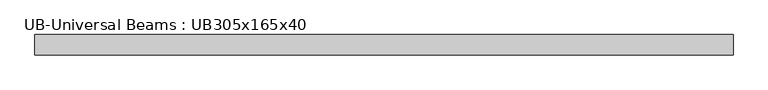
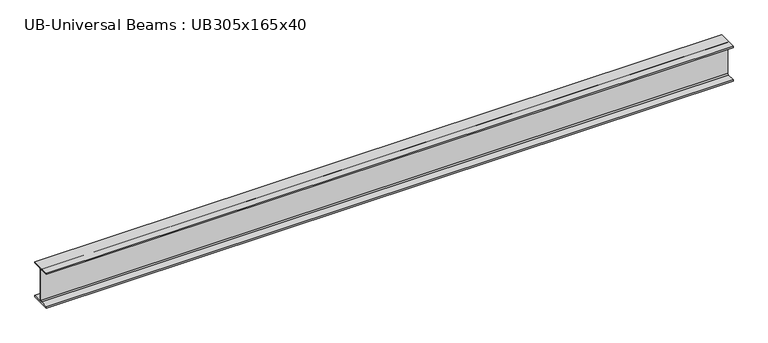
"""IFC4 building model written with IfcOpenShell, lengths in millimetres: beam geometry, UB-Universal Beams : UB305x165x40."""

from ifc_helpers import new_model, si_unit, point, frame, frame_2d, origin, place, context, project, spatial, polyline, circle_curve, trimmed, segment, composite_curve, outline, extrude, source, transform, mapped, element, save


def ub_universal_beams_ub305x165x40_7f5f946b(model_context):
    return source(origin(), model_context, "Body", "SweptSolid", [
        extrude(outline(composite_curve([segment(polyline([(82.5, -141.5), (82.5, -151.7), (-82.5, -151.7), (-82.5, -141.5), (-11.9, -141.5)]), True, "CONTINUOUS"), segment(trimmed(circle_curve(frame_2d((-11.9, -132.6)), 8.9), [point((-11.9, -141.5))], [point((-3.0, -132.6))], True, "CARTESIAN"), True, "CONTINUOUS"), segment(polyline([(-3.0, -132.6), (-3.0, 132.6)]), True, "CONTINUOUS"), segment(trimmed(circle_curve(frame_2d((-11.9, 132.6)), 8.9), [point((-3.0, 132.6))], [point((-11.9, 141.5))], True, "CARTESIAN"), True, "CONTINUOUS"), segment(polyline([(-11.9, 141.5), (-82.5, 141.5), (-82.5, 151.7), (82.5, 151.7), (82.5, 141.5), (11.9, 141.5)]), True, "CONTINUOUS"), segment(trimmed(circle_curve(frame_2d((11.9, 132.6)), 8.9), [point((11.9, 141.5))], [point((3.0, 132.6))], True, "CARTESIAN"), True, "CONTINUOUS"), segment(polyline([(3.0, 132.6), (3.0, -132.6)]), True, "CONTINUOUS"), segment(trimmed(circle_curve(frame_2d((11.9, -132.6)), 8.9), [point((3.0, -132.6))], [point((11.9, -141.5))], True, "CARTESIAN"), True, "CONTINUOUS"), segment(polyline([(11.9, -141.5), (82.5, -141.5)]), True, "CONTINUOUS")], self_intersect=False)), frame((-2833.3, 0.0, 0.0), z_axis=(1.0, 0.0, 0.0), x_axis=(0.0, 1.0, 0.0)), (0.0, 0.0, 1.0), 5666.6),
    ])


if __name__ == "__main__":
    model = new_model("IFC4")
    model_context = context("Model", 3, world=origin())
    ifc_project = project(units=[si_unit("LENGTHUNIT", "METRE", prefix="MILLI")], contexts=[model_context])
    site = spatial("IfcSite", under=ifc_project)
    building = spatial("IfcBuilding", under=site)
    placement = place(None, origin())
    ub_universal_beams_ub305x165x40_shape = ub_universal_beams_ub305x165x40_7f5f946b(model_context)
    element("IfcBeam", 1, ObjectType="UB-Universal Beams : UB305x165x40", at=placement, inside=building, context=model_context, shape_type="MappedRepresentation", body=[
        mapped(ub_universal_beams_ub305x165x40_shape, transform((0.0, 0.0, 0.0), x_axis=(1.0, 0.0, 0.0), y_axis=(0.0, 1.0, 0.0), z_axis=(0.0, 0.0, 1.0))),
    ])
    save(model, "model.ifc")

# Revit data of these elements
# Type "UB-Universal Beams : UB305x165x40"
#   Section Name Key = "UB305X165X40"
#   Width = 16.5 cm
#   Web Thickness = 0.6 cm
#   Web Fillet = 0.89 cm
#   Warping Constant = 164000.0 cm⁶
#   Torsional Moment of Inertia = 14.70 cm⁴
#   Section Area = 51.3 cm²
#   Plastic Modulus weak axis = 142.0 cm³
#   Plastic Modulus strong axis = 623.0 cm³
#   Nominal Weight = 40.2999 kgf/m
#   Moment of Inertia weak axis = 764.00 cm⁴
#   Moment of Inertia strong axis = 8503.00 cm⁴
#   Height = 30.34 cm
#   Flange Thickness = 1.02 cm
#   Elastic Modulus weak axis = 92.6 cm³
#   Elastic Modulus strong axis = 560.0 cm³
#   Centroid Vertical = 15.17 cm
#   Centroid Horizontal = 8.25 cm
#   Bolt Spacing = 9.0 cm
#   Length [instance default] = 1500 mm
#   Structural Material [instance default] = Metal - Steel 43-275
#   Type Comments = ""
#   Assembly Code = ""
# Element 1 (IfcBeam, "UB-Universal Beams : UB305x165x40")
#   Materials on its faces: "Metal - Steel 43-275"
# Materials
#   "Metal - Steel 43-275": class "Metal", colour RGB 247 247 247, transparency 0, Cost = 0
